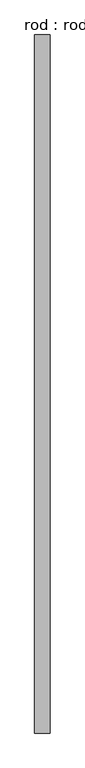
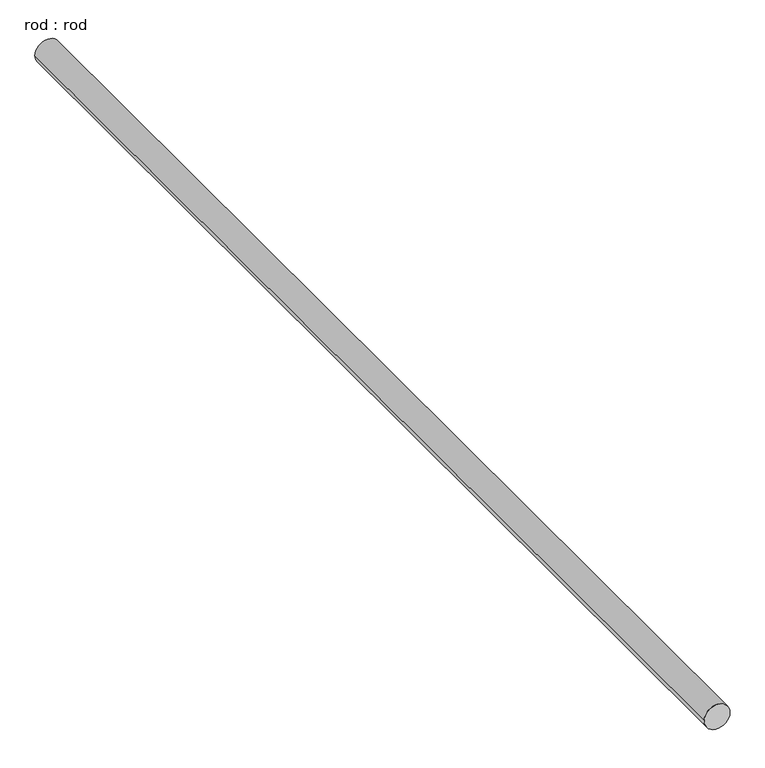
"""IFC4 building model written with IfcOpenShell, lengths in millimetres: proxy geometry, rod : rod."""

from ifc_helpers import new_model, si_unit, point, frame, frame_2d, origin, place, context, project, spatial, circle_curve, trimmed, segment, composite_curve, outline, extrude, source, transform, mapped, element, save


def rod_rod_a8c72223(model_context):
    return source(origin(), model_context, "Body", "SweptSolid", [
        extrude(outline(composite_curve([segment(trimmed(circle_curve(frame_2d((0.0108462, 0.0)), 200.0), [point((0.0108462, 200.0))], [point((0.0108462, -200.0))], False, "CARTESIAN"), True, "CONTINUOUS"), segment(trimmed(circle_curve(frame_2d((0.0108462, 0.0)), 200.0), [point((0.0108462, -200.0))], [point((0.0108462, 200.0))], False, "CARTESIAN"), True, "CONTINUOUS")], self_intersect=False)), frame((0.0, -4920.1094504, 0.0), z_axis=(0.0, 1.0, 0.0), x_axis=(0.0, 0.0, 1.0)), (0.0, 0.0, 1.0), 18025.6761316),
    ])


if __name__ == "__main__":
    model = new_model("IFC4")
    model_context = context("Model", 3, world=origin())
    ifc_project = project(units=[si_unit("LENGTHUNIT", "METRE", prefix="MILLI")], contexts=[model_context])
    site = spatial("IfcSite", under=ifc_project)
    building = spatial("IfcBuilding", under=site)
    placement = place(None, origin())
    rod_rod_shape = rod_rod_a8c72223(model_context)
    element("IfcBuildingElementProxy", 1, Name="rod : rod", ObjectType="rod : rod", at=placement, inside=building, context=model_context, shape_type="MappedRepresentation", body=[
        mapped(rod_rod_shape, transform((0.0, 0.0, 0.0), x_axis=(1.0, 0.0, 0.0), y_axis=(0.0, 1.0, 0.0), z_axis=(0.0, 0.0, 1.0))),
    ])
    save(model, "model.ifc")

# Revit data of these elements
# Type "rod : rod"
#   Default Elevation = 0
